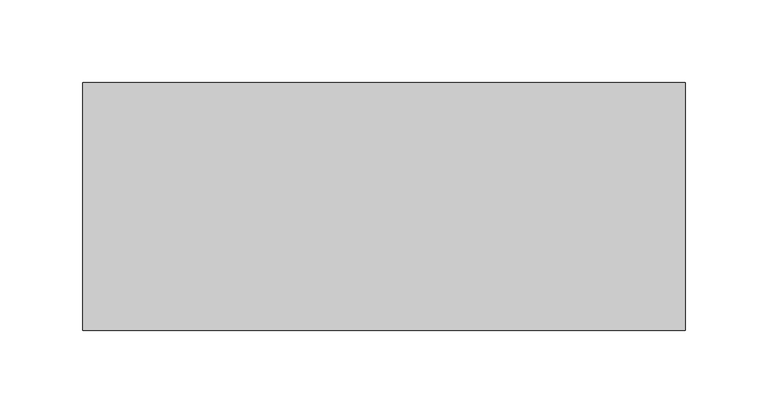
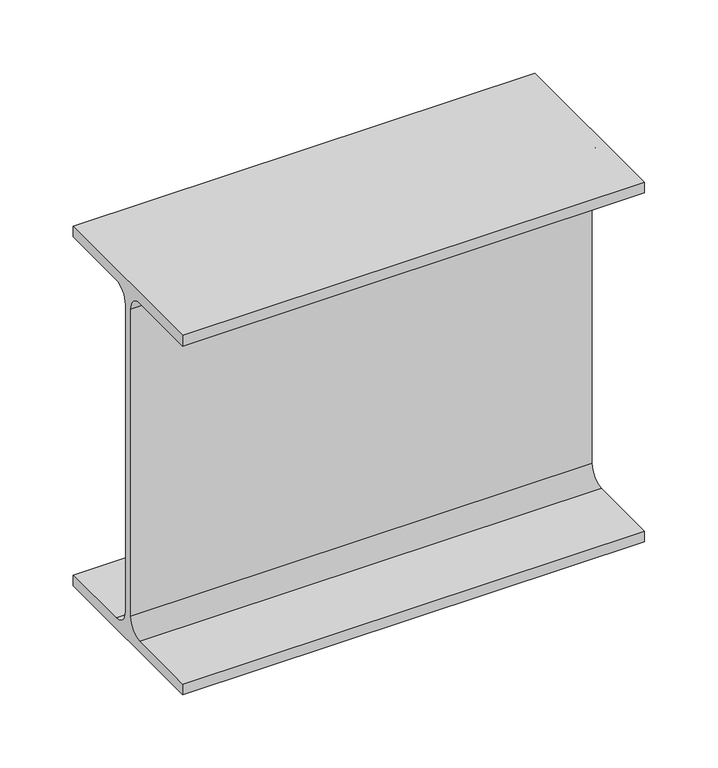
"""IFC4 building model written with IfcOpenShell, lengths in millimetres: beam geometry, 0912_Steel Framing_H-KSD3502 : H_SB_ASB_H-300x150x6.5x9."""

from ifc_helpers import new_model, si_unit, point, frame, frame_2d, origin, place, context, project, spatial, polyline, circle_curve, trimmed, segment, composite_curve, outline, extrude, source, transform, mapped, element, save


def beam_cad123e6(model_context):
    return source(origin(), model_context, "Body", "SweptSolid", [
        extrude(outline(composite_curve([segment(polyline([(75.0, -141.0), (75.0, -150.0), (-75.0, -150.0), (-75.0, -141.0), (-16.25, -141.0)]), True, "CONTINUOUS"), segment(trimmed(circle_curve(frame_2d((-16.25, -128.0)), 13.0), [point((-16.25, -141.0))], [point((-3.25, -128.0))], True, "CARTESIAN"), True, "CONTINUOUS"), segment(polyline([(-3.25, -128.0), (-3.25, 128.0)]), True, "CONTINUOUS"), segment(trimmed(circle_curve(frame_2d((-16.25, 128.0)), 13.0), [point((-3.25, 128.0))], [point((-16.25, 141.0))], True, "CARTESIAN"), True, "CONTINUOUS"), segment(polyline([(-16.25, 141.0), (-75.0, 141.0), (-75.0, 150.0), (75.0, 150.0), (75.0, 141.0), (16.25, 141.0)]), True, "CONTINUOUS"), segment(trimmed(circle_curve(frame_2d((16.25, 128.0)), 13.0), [point((16.25, 141.0))], [point((3.25, 128.0))], True, "CARTESIAN"), True, "CONTINUOUS"), segment(polyline([(3.25, 128.0), (3.25, -128.0)]), True, "CONTINUOUS"), segment(trimmed(circle_curve(frame_2d((16.25, -128.0)), 13.0), [point((3.25, -128.0))], [point((16.25, -141.0))], True, "CARTESIAN"), True, "CONTINUOUS"), segment(polyline([(16.25, -141.0), (75.0, -141.0)]), True, "CONTINUOUS")], self_intersect=False)), frame((-257.2999994, 0.0, 0.0), z_axis=(1.0, 0.0, 0.0), x_axis=(0.0, 1.0, 0.0)), (0.0, 0.0, 1.0), 364.5999994),
    ])


if __name__ == "__main__":
    model = new_model("IFC4")
    model_context = context("Model", 3, world=origin())
    ifc_project = project(units=[si_unit("LENGTHUNIT", "METRE", prefix="MILLI")], contexts=[model_context])
    site = spatial("IfcSite", under=ifc_project)
    building = spatial("IfcBuilding", under=site)
    placement = place(None, origin())
    beam_shape = beam_cad123e6(model_context)
    element("IfcBeam", 1, ObjectType="0912_Steel Framing_H-KSD3502 : H_SB_ASB_H-300x150x6.5x9", at=placement, inside=building, context=model_context, shape_type="MappedRepresentation", body=[
        mapped(beam_shape, transform((0.0, 0.0, 0.0), x_axis=(1.0, 0.0, 0.0), y_axis=(0.0, 1.0, 0.0), z_axis=(0.0, 0.0, 1.0))),
    ])
    save(model, "model.ifc")

# Revit data of these elements
# Type "0912_Steel Framing_H-KSD3502 : H_SB_ASB_H-300x150x6.5x9"
#   H_WM Code_1 = "S01AA002-00001 | Main Steel Structure Fabrication Work | Shelter/Building | Medium Steel - Standard (90KG/M>Weight≥30KG/M) | Material: (   )"
#   H_WM Code_2 = "S03AA028-00001 | Main Steel Structure Erection Work | Shelter/Building | Medium Steel (90KG/M>Weight≥30KG/M) | Material: (   )"
#   H_WM Code_3 = "S01AA010-00001 | Main Steel Structure Fabrication Work | Shelter/Building | Steel Painting/Coating | for Non-Fireproofed Steel Surface, Surface Preparation, Primer, Second & Final Coat | Material: (   )"
#   H_Q'ty Cal Type Tag = "SB-Q2"
#   Width = 15.0 cm
#   Web Thickness = 0.65 cm
#   Web Fillet = 1.3 cm
#   Warping Constant = 107000.0 cm⁶
#   W = 0
#   Torsional Moment of Inertia = 9.9539 cm⁴
#   Section Area = 46.78 cm²
#   Plastic Modulus weak axis = 105.0 cm³
#   Plastic Modulus strong axis = 542.0 cm³
#   Perimeter = 1.17 m²/m
#   Nominal Weight = 36.70 kgf/m
#   Moment of Inertia weak axis = 508.00 cm⁴
#   Moment of Inertia strong axis = 7210.00 cm⁴
#   Height = 30.0 cm
#   Flange Thickness = 0.9 cm
#   Elastic Modulus weak axis = 67.7 cm³
#   Elastic Modulus strong axis = 481.0 cm³
#   Centroid Vertical = 15.0 cm
#   Centroid Horizontal = 7.5 cm
#   Ix = 72100000
#   Length [instance default] = 1.5240 m
#   Zx = 542000
#   b = 0.1500 m
#   h = 0.3000 m
#   r = 0.0130 m
#   s = 0.0065 m
#   t = 0.0090 m
#   A = 0.004678 m²
#   Structural Material [instance default] = Steel, 45-345
#   Assembly Code = ""
# Element 1 (IfcBeam, "0912_Steel Framing_H-KSD3502 : H_SB_ASB_H-300x150x6.5x9")
#   Structural Material = none
# Materials
#   "Steel, 45-345": class "Metal", colour RGB 189 187 185, transparency 0, Description = "Steel 345 MPa", Cost = 0
